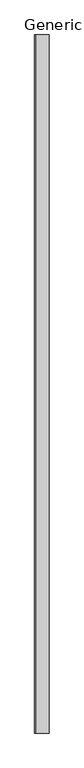
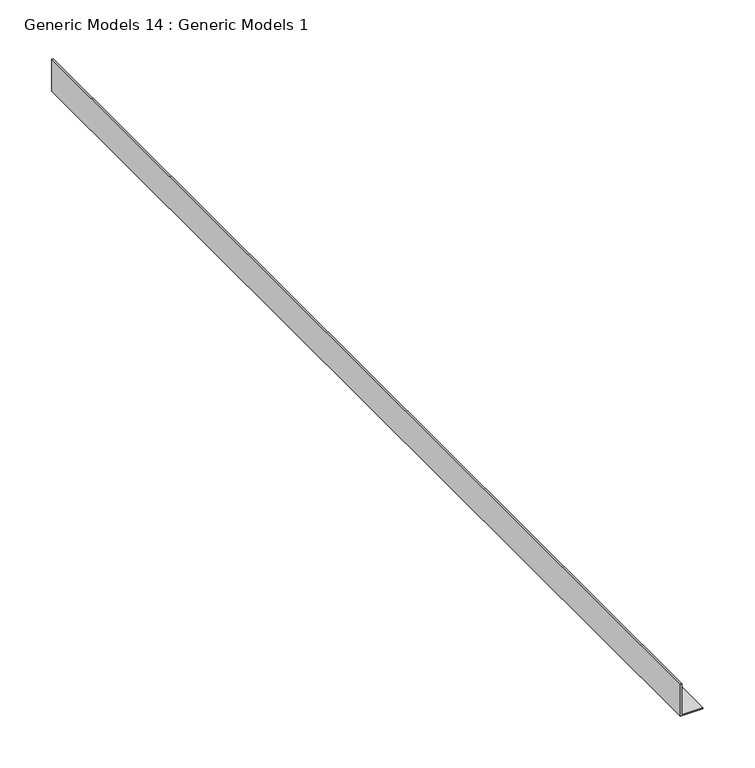
"""IFC4 building model written with IfcOpenShell, lengths in millimetres: proxy geometry, Generic Models 14 : Generic Models 1."""

from ifc_helpers import new_model, si_unit, frame, origin, place, context, project, spatial, polyline, outline, extrude, source, transform, mapped, element, save


def generic_models_14_generic_models_1_e8c90d4c(model_context):
    return source(origin(), model_context, "Body", "SweptSolid", [
        extrude(outline(polyline([(2277.1204978, 49799.875), (2239.0204978, 49799.875), (2239.0204978, 49825.275), (2240.6079978, 49825.275), (2240.6079978, 49801.4625), (2277.1204978, 49801.4625), (2277.1204978, 49799.875)])), frame((0.0, 0.0, 0.0), z_axis=(0.0, 1.0, 0.0), x_axis=(0.0, 0.0, 1.0)), (0.0, 0.0, 1.0), 1219.2),
    ])


if __name__ == "__main__":
    model = new_model("IFC4")
    model_context = context("Model", 3, world=origin())
    ifc_project = project(units=[si_unit("LENGTHUNIT", "METRE", prefix="MILLI")], contexts=[model_context])
    site = spatial("IfcSite", under=ifc_project)
    building = spatial("IfcBuilding", under=site)
    placement = place(None, origin())
    generic_models_14_generic_models_1_shape = generic_models_14_generic_models_1_e8c90d4c(model_context)
    element("IfcBuildingElementProxy", 1, Name="Generic Models 14 : Generic Models 1", ObjectType="Generic Models 14 : Generic Models 1", at=placement, inside=building, context=model_context, shape_type="MappedRepresentation", body=[
        mapped(generic_models_14_generic_models_1_shape, transform((0.0, 0.0, 0.0), x_axis=(1.0, 0.0, 0.0), y_axis=(0.0, 1.0, 0.0), z_axis=(0.0, 0.0, 1.0))),
    ])
    save(model, "model.ifc")

# Revit data of these elements
# Element 1 (IfcBuildingElementProxy, "Generic Models 14 : Generic Models 1")
#   Materials on its faces: "CEILING TRACK AS SCHEDULED"
# Materials
#   "CEILING TRACK AS SCHEDULED": class "Unassigned", colour RGB 210 209 208, transparency 0, Keynote = "M05121300.02", Cost = 0
